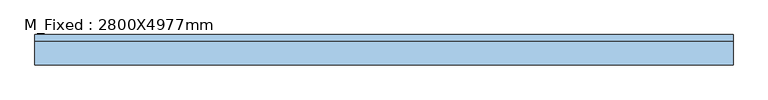
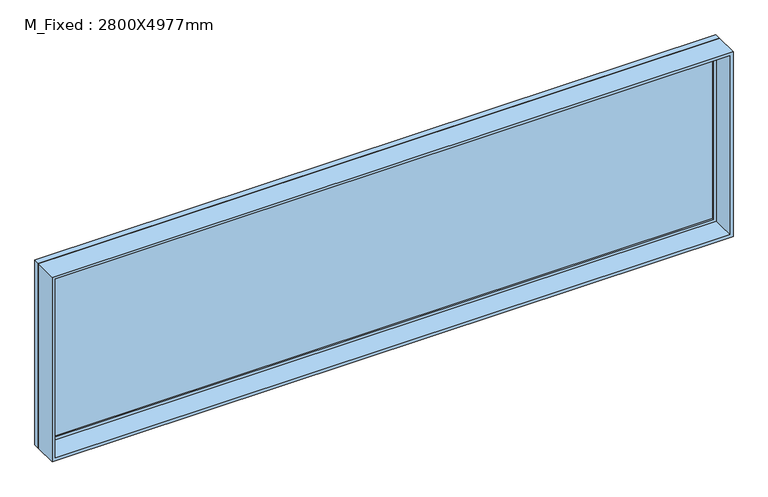
"""IFC4 building model written with IfcOpenShell, lengths in millimetres: window geometry, M_Fixed : 2800X4977mm."""

import ifcopenshell
import ifcopenshell.guid

model = None  # the IFC model being written
_history = None  # IfcOwnerHistory: only IFC2X3 demands one
_inside = {}  # id of a spatial element -> (the spatial element, [elements in it])
_under = {}  # id of a project, library or spatial element -> (it, [spatial elements below it])
_declared = {}  # id of a project -> (the project, [libraries it declares])
_typed = {}  # id of a type object -> (the type object, [elements of that type])
_made_of = {}  # id of a material, layer set ... -> (it, [elements and type objects made of it])


def new_model(schema):
    """Start an empty IFC model of exactly this schema.

    Asked for "IFC4X3", IfcOpenShell would pick the latest addendum, in which some entities
    have other attributes; the version numbers below select the first issue.
    IFC2X3 requires an IfcOwnerHistory on every rooted entity: one is made here for all.
    """
    global model, _history
    if schema == "IFC4X3":
        model = ifcopenshell.file(schema_version=(4, 3, 0, 0))
    else:
        model = ifcopenshell.file(schema=schema)
    _inside.clear()
    _under.clear()
    _declared.clear()
    _typed.clear()
    _made_of.clear()
    _history = None
    if model.schema == "IFC2X3":
        org = make("IfcOrganization", Name="unknown")
        user = make(
            "IfcPersonAndOrganization",
            ThePerson=make("IfcPerson", FamilyName="unknown"),
            TheOrganization=org,
        )
        app = make(
            "IfcApplication",
            ApplicationDeveloper=org,
            Version="unknown",
            ApplicationFullName="unknown",
            ApplicationIdentifier="unknown",
        )
        _history = make(
            "IfcOwnerHistory",
            OwningUser=user,
            OwningApplication=app,
            ChangeAction="ADDED",
            CreationDate=0,
        )
    return model


def make(cls, **values):
    """One entity of the class cls with the attributes given. An attribute that is None is left unset."""
    return model.create_entity(
        cls, **{name: value for name, value in values.items() if value is not None}
    )


def rooted(cls, **values):
    """An entity with a GlobalId (a new one), such as an element, a storey or a relation."""
    return make(cls, GlobalId=ifcopenshell.guid.new(), OwnerHistory=_history, **values)


def si_unit(unit_type, name, prefix=None):
    """IfcSIUnit, for example si_unit("LENGTHUNIT", "METRE", prefix="MILLI")."""
    return make("IfcSIUnit", UnitType=unit_type, Prefix=prefix, Name=name)


def assignment(units):
    """IfcUnitAssignment: the units of a project."""
    return None if units is None else make("IfcUnitAssignment", Units=units)


def point(xyz):
    """IfcCartesianPoint."""
    return None if xyz is None else make("IfcCartesianPoint", Coordinates=xyz)


def direction(xyz):
    """IfcDirection."""
    return None if xyz is None else make("IfcDirection", DirectionRatios=xyz)


def frame(location, z_axis=None, x_axis=None):
    """IfcAxis2Placement3D, a coordinate frame: its origin and axes. An axis left out is left unset."""
    return make(
        "IfcAxis2Placement3D",
        Location=point(location),
        Axis=direction(z_axis),
        RefDirection=direction(x_axis),
    )


def origin():
    """The frame at (0, 0, 0) with its axes left unset."""
    return frame((0.0, 0.0, 0.0))


def place(relative_to, where):
    """IfcLocalPlacement: puts the frame where relative to a parent placement (None: the world)."""
    return make(
        "IfcLocalPlacement", PlacementRelTo=relative_to, RelativePlacement=where
    )


def context(
    kind, dimensions, precision=None, world=None, true_north=None, identifier=None
):
    """IfcGeometricRepresentationContext, for example the 3D "Model" context."""
    return make(
        "IfcGeometricRepresentationContext",
        ContextIdentifier=identifier,
        ContextType=kind,
        CoordinateSpaceDimension=dimensions,
        Precision=precision,
        WorldCoordinateSystem=world,
        TrueNorth=true_north,
    )


def project(units=None, contexts=None):
    """IfcProject with its units and contexts."""
    return rooted(
        "IfcProject",
        Name="project",
        RepresentationContexts=contexts,
        UnitsInContext=assignment(units),
    )


def spatial(cls, under=None, at=None, **own):
    """A site, building, storey or space (cls), placed at a placement, below another one or the project."""
    s = rooted(cls, ObjectPlacement=at, **own)
    if under is not None:
        _under.setdefault(under.id(), (under, []))[1].append(s)
    return s


def polyline(points):
    """IfcPolyline through the points."""
    return make("IfcPolyline", Points=[point(p) for p in points])


def outline(outer, holes=None, kind="AREA"):
    """IfcArbitraryClosedProfileDef: a profile drawn as a closed curve; with holes, ...WithVoids."""
    if holes is None:
        return make("IfcArbitraryClosedProfileDef", ProfileType=kind, OuterCurve=outer)
    return make(
        "IfcArbitraryProfileDefWithVoids",
        ProfileType=kind,
        OuterCurve=outer,
        InnerCurves=holes,
    )


def extrude(swept, where, along, depth):
    """IfcExtrudedAreaSolid: the profile swept, set in the frame where, extruded along a direction by depth."""
    return make(
        "IfcExtrudedAreaSolid",
        SweptArea=swept,
        Position=where,
        ExtrudedDirection=direction(along),
        Depth=depth,
    )


def shape(context_of_items, identifier, shape_type, items):
    """IfcShapeRepresentation: the items that make up one representation, for example the "Body"."""
    return make(
        "IfcShapeRepresentation",
        ContextOfItems=context_of_items,
        RepresentationIdentifier=identifier,
        RepresentationType=shape_type,
        Items=items,
    )


def source(mapping_origin, context_of_items, identifier, shape_type, items):
    """IfcRepresentationMap: a shape defined once, which mapped items show again and again."""
    return make(
        "IfcRepresentationMap",
        MappingOrigin=mapping_origin,
        MappedRepresentation=shape(context_of_items, identifier, shape_type, items),
    )


def transform(
    local_origin,
    x_axis=None,
    y_axis=None,
    z_axis=None,
    scale=None,
    scale2=None,
    scale3=None,
    uniform=True,
):
    """IfcCartesianTransformationOperator3D, or its non-uniform kind. x_axis, y_axis, z_axis: its Axis1, 2, 3."""
    if uniform:
        return make(
            "IfcCartesianTransformationOperator3D",
            Axis1=direction(x_axis),
            Axis2=direction(y_axis),
            LocalOrigin=point(local_origin),
            Scale=scale,
            Axis3=direction(z_axis),
        )
    return make(
        "IfcCartesianTransformationOperator3DnonUniform",
        Axis1=direction(x_axis),
        Axis2=direction(y_axis),
        LocalOrigin=point(local_origin),
        Scale=scale,
        Axis3=direction(z_axis),
        Scale2=scale2,
        Scale3=scale3,
    )


def mapped(mapping_source, mapping_target):
    """IfcMappedItem: shows the shape of a source again, moved by a transform."""
    return make(
        "IfcMappedItem", MappingSource=mapping_source, MappingTarget=mapping_target
    )


def made_of(thing, what):
    """Note that an element or type object is made of a material, layer set ...; save() writes the relation."""
    if what is not None:
        _made_of.setdefault(what.id(), (what, []))[1].append(thing)
    return thing


def element(
    cls,
    number,
    at=None,
    inside=None,
    cuts=None,
    type_object=None,
    material=None,
    context=None,
    identifier="Body",
    shape_type=None,
    held_by="IfcProductDefinitionShape",
    body=None,
    shapes=None,
    **own,
):
    """One element of the class cls, such as IfcWall. Its Tag is "e" and its number.

    at: its placement. inside: the storey or other place that contains it. cuts: it is an
    opening in that element (IfcRelVoidsElement). A single representation is given by context,
    identifier, shape_type and body (its items); several are given by shapes. held_by: the class
    of the entity that holds the representations. save() writes the other relations.
    """
    e = rooted(cls, Tag="e%d" % number, ObjectPlacement=at, **own)
    if body is not None:
        shapes = [shape(context, identifier, shape_type, body)]
    if shapes is not None:
        e.Representation = make(held_by, Representations=shapes)
    if inside is not None:
        _inside.setdefault(inside.id(), (inside, []))[1].append(e)
    if cuts is not None:
        rooted(
            "IfcRelVoidsElement", RelatingBuildingElement=cuts, RelatedOpeningElement=e
        )
    if type_object is not None:
        _typed.setdefault(type_object.id(), (type_object, []))[1].append(e)
    return made_of(e, material)


def aggregate(whole, parts):
    """IfcRelAggregates: a whole, such as a stair, and the parts it consists of."""
    return rooted("IfcRelAggregates", RelatingObject=whole, RelatedObjects=parts)


def save(model, path):
    """Write the relations noted so far, then the file.

    IfcRelAggregates (storeys below a building ...), IfcRelContainedInSpatialStructure (elements
    in a storey), IfcRelDefinesByType, IfcRelAssociatesMaterial and IfcRelDeclares: one each for
    every whole, place, type object, material and project.
    """
    for whole, parts in _under.values():
        aggregate(whole, parts)
    for where, things in _inside.values():
        rooted(
            "IfcRelContainedInSpatialStructure",
            RelatedElements=things,
            RelatingStructure=where,
        )
    for kind, things in _typed.values():
        rooted("IfcRelDefinesByType", RelatedObjects=things, RelatingType=kind)
    for what, things in _made_of.values():
        rooted("IfcRelAssociatesMaterial", RelatedObjects=things, RelatingMaterial=what)
    for by, libraries in _declared.values():
        rooted("IfcRelDeclares", RelatingContext=by, RelatedDefinitions=libraries)
    model.write(path)


def m_fixed_2800x4977mm_04857461(model_context):
    return source(origin(), model_context, "Body", "SweptSolid", [
        extrude(outline(polyline([(-3420.85, 130.4), (3420.85, 130.4), (3420.85, 118.4), (-3420.85, 118.4), (-3420.85, 130.4)])), frame((0.0, 0.0, 978.0), z_axis=(0.0, 0.0, 1.0), x_axis=(1.0, 0.0, 0.0)), (0.0, 0.0, 1.0), 1874.0),
        extrude(outline(polyline([(2896.0, -3464.85), (934.0, -3464.85), (934.0, 3464.85), (2896.0, 3464.85), (2896.0, -3464.85)]), holes=[polyline([(2852.0, -3420.85), (2852.0, 3420.85), (978.0, 3420.85), (978.0, -3420.85), (2852.0, -3420.85)])]), frame((0.0, 102.4, 0.0), z_axis=(0.0, 1.0, 0.0), x_axis=(0.0, 0.0, 1.0)), (0.0, 0.0, 1.0), 44.0),
        extrude(outline(polyline([(2915.0, -3483.85), (915.0, -3483.85), (915.0, 3483.85), (2915.0, 3483.85), (2915.0, -3483.85)]), holes=[polyline([(2896.0, -3464.85), (2896.0, 3464.85), (934.0, 3464.85), (934.0, -3464.85), (2896.0, -3464.85)])]), frame((0.0, 102.4, 0.0), z_axis=(0.0, 1.0, 0.0), x_axis=(0.0, 0.0, 1.0)), (0.0, 0.0, 1.0), 63.0),
        extrude(outline(polyline([(2915.0, -3483.85), (915.0, -3483.85), (915.0, 3483.85), (2915.0, 3483.85), (2915.0, -3483.85)]), holes=[polyline([(2883.0, -3451.85), (2883.0, 3451.85), (947.0, 3451.85), (947.0, -3451.85), (2883.0, -3451.85)])]), frame((0.0, -139.4, 0.0), z_axis=(0.0, 1.0, 0.0), x_axis=(0.0, 0.0, 1.0)), (0.0, 0.0, 1.0), 241.8),
    ])


if __name__ == "__main__":
    model = new_model("IFC4")
    model_context = context("Model", 3, world=origin())
    ifc_project = project(units=[si_unit("LENGTHUNIT", "METRE", prefix="MILLI")], contexts=[model_context])
    site = spatial("IfcSite", under=ifc_project)
    building = spatial("IfcBuilding", under=site)
    placement = place(None, origin())
    m_fixed_2800x4977mm_shape = m_fixed_2800x4977mm_04857461(model_context)
    element("IfcWindow", 1, ObjectType="M_Fixed : 2800X4977mm", at=placement, inside=building, context=model_context, shape_type="MappedRepresentation", body=[
        mapped(m_fixed_2800x4977mm_shape, transform((0.0, 0.0, 0.0), x_axis=(1.0, 0.0, 0.0), y_axis=(0.0, 1.0, 0.0), z_axis=(0.0, 0.0, 1.0))),
    ])
    save(model, "model.ifc")

# Revit data of these elements
# Type "M_Fixed : 2800X4977mm"
#   Type Mark = "29"
#   Height = 2000 mm
#   Default Sill Height = 915 mm
#   Width = 6967.7 mm
#   Window Inset = 19 mm
#   Frame Exterior Material = Sash
#   Frame Interior Material = Sash
#   Glass Pane Material = Glass
#   Sash = Sash
#   Wall Closure = (empty or 0)
# Element 1 (IfcWindow, "M_Fixed : 2800X4977mm")
#   Materials on its faces: "Sash", "Glass"
# Materials
#   "Sash": class "Wood", colour RGB 136 99 55, transparency 0
#   "Glass": class "Glass", colour RGB 0 128 192, transparency 0.9, Description = "Soda Lime Glass", Cost = 0
